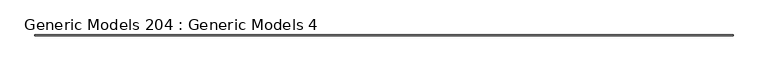
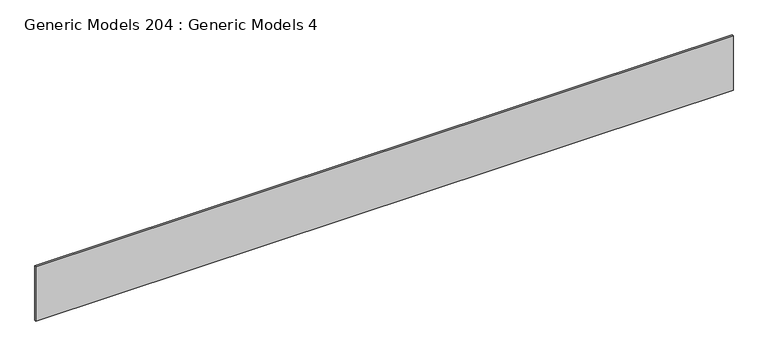
"""IFC4 building model written with IfcOpenShell, lengths in millimetres: proxy geometry, Generic Models 204 : Generic Models 4."""

from ifc_helpers import new_model, si_unit, frame, origin, place, context, project, spatial, polyline, outline, extrude, source, transform, mapped, element, save


def generic_models_204_generic_models_4_4a2e1d4b(model_context):
    return source(origin(), model_context, "Body", "SweptSolid", [
        extrude(outline(polyline([(-8500.0048466, -29089.2060818), (-8500.0048466, -29108.2560818), (-20795.7733045, -29108.2560818), (-20795.7733045, -29089.2060818), (-8500.0048466, -29089.2060818)])), frame((0.0, 0.0, 125487.5242553), z_axis=(0.0, 0.0, 1.0), x_axis=(1.0, 0.0, 0.0)), (0.0, 0.0, 1.0), 1015.5696958),
    ])


if __name__ == "__main__":
    model = new_model("IFC4")
    model_context = context("Model", 3, world=origin())
    ifc_project = project(units=[si_unit("LENGTHUNIT", "METRE", prefix="MILLI")], contexts=[model_context])
    site = spatial("IfcSite", under=ifc_project)
    building = spatial("IfcBuilding", under=site)
    placement = place(None, origin())
    generic_models_204_generic_models_4_shape = generic_models_204_generic_models_4_4a2e1d4b(model_context)
    element("IfcBuildingElementProxy", 1, Name="Generic Models 204 : Generic Models 4", ObjectType="Generic Models 204 : Generic Models 4", at=placement, inside=building, context=model_context, shape_type="MappedRepresentation", body=[
        mapped(generic_models_204_generic_models_4_shape, transform((0.0, 0.0, 0.0), x_axis=(1.0, 0.0, 0.0), y_axis=(0.0, 1.0, 0.0), z_axis=(0.0, 0.0, 1.0))),
    ])
    save(model, "model.ifc")

# Revit data of these elements
# Element 1 (IfcBuildingElementProxy, "Generic Models 204 : Generic Models 4")
#   Materials on its faces: "_CDX PLYWOOD - SEE STRUCT DWGs"
# Materials
#   "_CDX PLYWOOD - SEE STRUCT DWGs": class "Generic", colour RGB 98 75 74, transparency 0, Cost = 0
